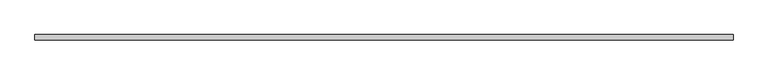
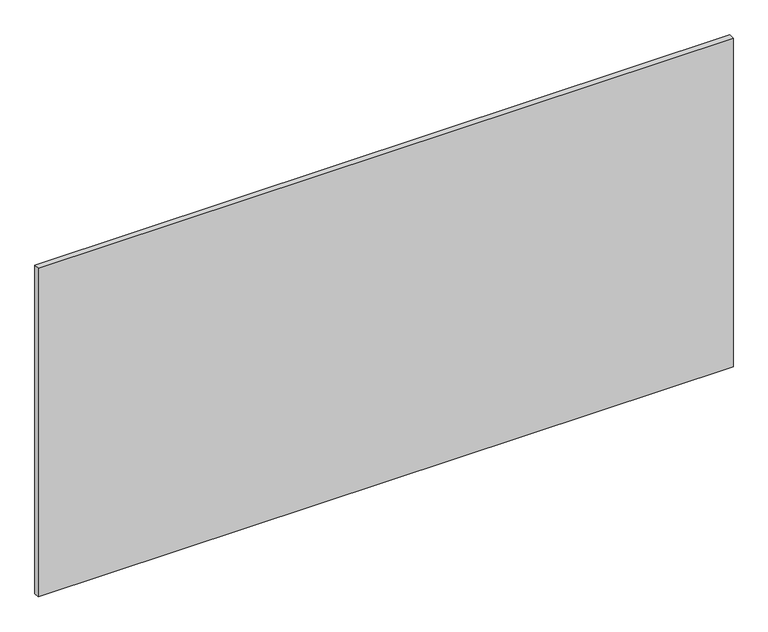
"""IFC4 building model written with IfcOpenShell, lengths in millimetres: proxy geometry, Inner panel:Inner panel:1:Inner panel:1 : Inner panel:Inner panel:300324:3:Inner panel:1:Inner panel:1 : Inner panel:Inner panel:300324:3 : Inner panel:Inner panel:1:Inner panel:1 : Inner panel:Inner panel:300324:300043:1 : Inner panel:Inner panel:1:Inner panel:1 : Inner panel:Inner panel:300324:3:Inner panel:1:Inner panel:1 : Inner panel:Inner panel:300324:3 : Inner panel:Inner panel:1:Inner panel:1 : Inner panel:Inner panel:300324:300043:310272."""

from ifc_helpers import new_model, si_unit, frame, origin, place, context, project, spatial, polyline, outline, extrude, source, transform, mapped, element, save


def generic_models_25eaa928(model_context):
    return source(origin(), model_context, "Body", "SweptSolid", [
        extrude(outline(polyline([(591286.9867242, -536830.3413358), (591286.9867242, -536811.2913358), (593725.3867242, -536811.2913358), (593725.3867242, -536830.3413358), (591286.9867242, -536830.3413358)])), frame((0.0, 0.0, 2495.55), z_axis=(0.0, 0.0, 1.0), x_axis=(1.0, 0.0, 0.0)), (0.0, 0.0, 1.0), 1219.2),
    ])


if __name__ == "__main__":
    model = new_model("IFC4")
    model_context = context("Model", 3, world=origin())
    ifc_project = project(units=[si_unit("LENGTHUNIT", "METRE", prefix="MILLI")], contexts=[model_context])
    site = spatial("IfcSite", under=ifc_project)
    building = spatial("IfcBuilding", under=site)
    placement = place(None, origin())
    generic_models_shape = generic_models_25eaa928(model_context)
    element("IfcBuildingElementProxy", 1, Name="Inner panel:Inner panel:1:Inner panel:1 : Inner panel:Inner panel:300324:3:Inner panel:1:Inner panel:1 : Inner panel:Inner panel:300324:3 : Inner panel:Inner panel:1:Inner panel:1 : Inner panel:Inner panel:300324:300043:1 : Inner panel:Inner panel:1:Inner panel:1 : Inner panel:Inner panel:300324:3:Inner panel:1:Inner panel:1 : Inner panel:Inner panel:300324:3 : Inner panel:Inner panel:1:Inner panel:1 : Inner panel:Inner panel:300324:300043:310272", ObjectType="Inner panel:Inner panel:1:Inner panel:1 : Inner panel:Inner panel:300324:3:Inner panel:1:Inner panel:1 : Inner panel:Inner panel:300324:3 : Inner panel:Inner panel:1:Inner panel:1 : Inner panel:Inner panel:300324:300043:1 : Inner panel:Inner panel:1:Inner panel:1 : Inner panel:Inner panel:300324:3:Inner panel:1:Inner panel:1 : Inner panel:Inner panel:300324:3 : Inner panel:Inner panel:1:Inner panel:1 : Inner panel:Inner panel:300324:300043:310272", at=placement, inside=building, context=model_context, shape_type="MappedRepresentation", body=[
        mapped(generic_models_shape, transform((0.0, 0.0, 0.0), x_axis=(1.0, 0.0, 0.0), y_axis=(0.0, 1.0, 0.0), z_axis=(0.0, 0.0, 1.0))),
    ])
    save(model, "model.ifc")

# Revit data of these elements
# Type "Inner panel:Inner panel:1:Inner panel:1 : Inner panel:Inner panel:300324:3:Inner panel:1:Inner panel:1 : Inner panel:Inner panel:300324:3 : Inner panel:Inner panel:1:Inner panel:1 : Inner panel:Inner panel:300324:300043:1 : Inner panel:Inner panel:1:Inner panel:1 : Inner panel:Inner panel:300324:3:Inner panel:1:Inner panel:1 : Inner panel:Inner panel:300324:3 : Inner panel:Inner panel:1:Inner panel:1 : Inner panel:Inner panel:300324:300043:310272"
#   NameOverride = "Inner panel:Inner panel:1:Inner panel:1 : Inner panel:Inner panel:300324:3:Inner panel:1:Inner panel:1 : Inner panel:Inner panel:300324:3 : Inner panel:Inner panel:1:Inner panel:1 : Inner panel:Inner panel:300324:300043:310272"
#   ObjectTypeOverride = "Inner panel:1:Inner panel:1 : Inner panel:Inner panel:300324:3 : Inner panel:Inner panel:1:Inner panel:1 : Inner panel:Inner panel:300324:300043"
#   Reference = "Inner panel"
#   Tag = "310272"
# Element 1 (IfcBuildingElementProxy, "Inner panel:Inner panel:1:Inner panel:1 : Inner panel:Inner panel:300324:3:Inner panel:1:Inner panel:1 : Inner panel:Inner panel:300324:3 : Inner panel:Inner panel:1:Inner panel:1 : Inner panel:Inner panel:300324:300043:1 : Inner panel:Inner panel:1:Inner panel:1 : Inner panel:Inner panel:300324:3:Inner panel:1:Inner panel:1 : Inner panel:Inner panel:300324:3 : Inner panel:Inner panel:1:Inner panel:1 : Inner panel:Inner panel:300324:300043:310272")
#   Materials on its faces: "¾” (CLASS A) FIRE RETARDANT PLYWOOD ...OR… IF 1/4\" GYP. BD UNDER PLYWOOD, FLAME SPREAD TO BE CLASS C -  (FINISH: GRADE B - PREFINISHED STAINED/SEALED) - 1/4\" GAP BTWN PANELS (FASTENERS T.B.D.)"
# Materials
#   "¾” (CLASS A) FIRE RETARDANT PLYWOOD ...OR… IF 1/4\" GYP. BD UNDER PLYWOOD, FLAME SPREAD TO BE CLASS C -  (FINISH: GRADE B - PREFINISHED STAINED/SEALED) - 1/4\" GAP BTWN PANELS (FASTENERS T.B.D.)": class "Wood", colour RGB 149 120 74, transparency 0, Description = "Plywood, sheathing grade", Cost = 0
